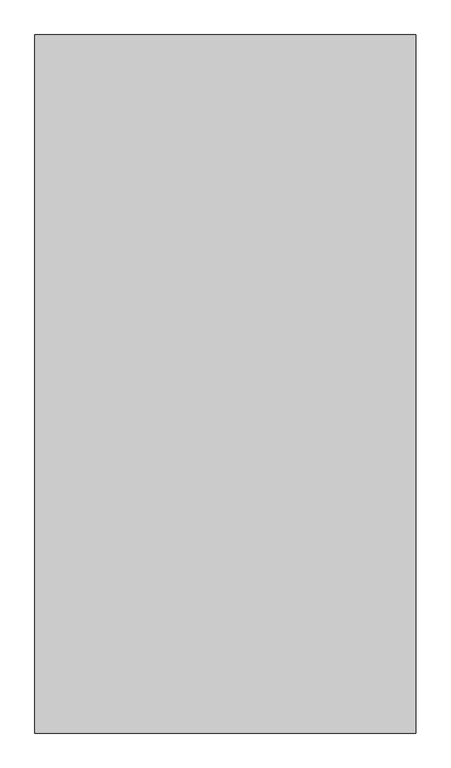
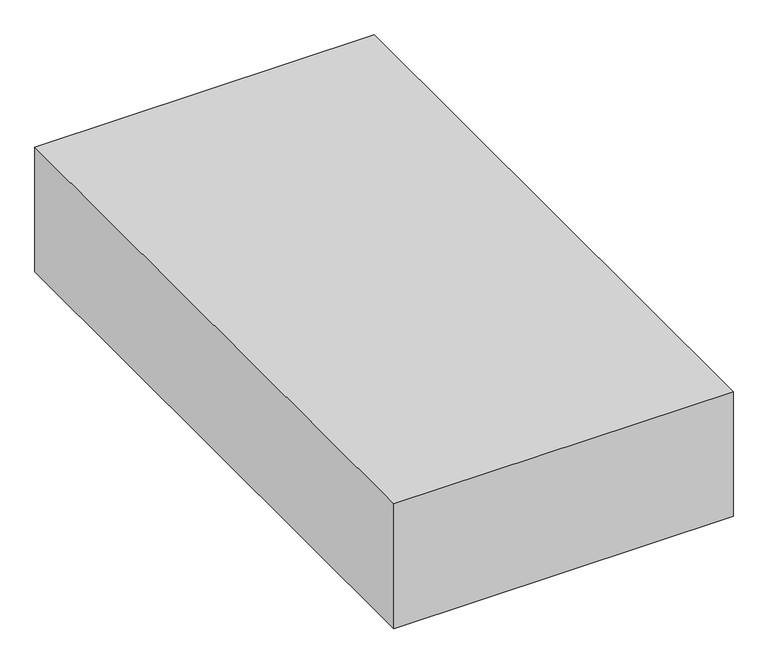
"""IFC4 building model written with IfcOpenShell, lengths in millimetres: proxy geometry, Space Planning Box_hec : Space Planning Box_hec."""

import ifcopenshell
import ifcopenshell.guid

model = None  # the IFC model being written
_history = None  # IfcOwnerHistory: only IFC2X3 demands one
_inside = {}  # id of a spatial element -> (the spatial element, [elements in it])
_under = {}  # id of a project, library or spatial element -> (it, [spatial elements below it])
_declared = {}  # id of a project -> (the project, [libraries it declares])
_typed = {}  # id of a type object -> (the type object, [elements of that type])
_made_of = {}  # id of a material, layer set ... -> (it, [elements and type objects made of it])


def new_model(schema):
    """Start an empty IFC model of exactly this schema.

    Asked for "IFC4X3", IfcOpenShell would pick the latest addendum, in which some entities
    have other attributes; the version numbers below select the first issue.
    IFC2X3 requires an IfcOwnerHistory on every rooted entity: one is made here for all.
    """
    global model, _history
    if schema == "IFC4X3":
        model = ifcopenshell.file(schema_version=(4, 3, 0, 0))
    else:
        model = ifcopenshell.file(schema=schema)
    _inside.clear()
    _under.clear()
    _declared.clear()
    _typed.clear()
    _made_of.clear()
    _history = None
    if model.schema == "IFC2X3":
        org = make("IfcOrganization", Name="unknown")
        user = make(
            "IfcPersonAndOrganization",
            ThePerson=make("IfcPerson", FamilyName="unknown"),
            TheOrganization=org,
        )
        app = make(
            "IfcApplication",
            ApplicationDeveloper=org,
            Version="unknown",
            ApplicationFullName="unknown",
            ApplicationIdentifier="unknown",
        )
        _history = make(
            "IfcOwnerHistory",
            OwningUser=user,
            OwningApplication=app,
            ChangeAction="ADDED",
            CreationDate=0,
        )
    return model


def make(cls, **values):
    """One entity of the class cls with the attributes given. An attribute that is None is left unset."""
    return model.create_entity(
        cls, **{name: value for name, value in values.items() if value is not None}
    )


def rooted(cls, **values):
    """An entity with a GlobalId (a new one), such as an element, a storey or a relation."""
    return make(cls, GlobalId=ifcopenshell.guid.new(), OwnerHistory=_history, **values)


def si_unit(unit_type, name, prefix=None):
    """IfcSIUnit, for example si_unit("LENGTHUNIT", "METRE", prefix="MILLI")."""
    return make("IfcSIUnit", UnitType=unit_type, Prefix=prefix, Name=name)


def assignment(units):
    """IfcUnitAssignment: the units of a project."""
    return None if units is None else make("IfcUnitAssignment", Units=units)


def point(xyz):
    """IfcCartesianPoint."""
    return None if xyz is None else make("IfcCartesianPoint", Coordinates=xyz)


def direction(xyz):
    """IfcDirection."""
    return None if xyz is None else make("IfcDirection", DirectionRatios=xyz)


def frame(location, z_axis=None, x_axis=None):
    """IfcAxis2Placement3D, a coordinate frame: its origin and axes. An axis left out is left unset."""
    return make(
        "IfcAxis2Placement3D",
        Location=point(location),
        Axis=direction(z_axis),
        RefDirection=direction(x_axis),
    )


def origin():
    """The frame at (0, 0, 0) with its axes left unset."""
    return frame((0.0, 0.0, 0.0))


def origin_with_axes():
    """The frame at (0, 0, 0) with the z axis (0, 0, 1) and the x axis (1, 0, 0) written out."""
    return frame((0.0, 0.0, 0.0), z_axis=(0.0, 0.0, 1.0), x_axis=(1.0, 0.0, 0.0))


def place(relative_to, where):
    """IfcLocalPlacement: puts the frame where relative to a parent placement (None: the world)."""
    return make(
        "IfcLocalPlacement", PlacementRelTo=relative_to, RelativePlacement=where
    )


def context(
    kind, dimensions, precision=None, world=None, true_north=None, identifier=None
):
    """IfcGeometricRepresentationContext, for example the 3D "Model" context."""
    return make(
        "IfcGeometricRepresentationContext",
        ContextIdentifier=identifier,
        ContextType=kind,
        CoordinateSpaceDimension=dimensions,
        Precision=precision,
        WorldCoordinateSystem=world,
        TrueNorth=true_north,
    )


def project(units=None, contexts=None):
    """IfcProject with its units and contexts."""
    return rooted(
        "IfcProject",
        Name="project",
        RepresentationContexts=contexts,
        UnitsInContext=assignment(units),
    )


def spatial(cls, under=None, at=None, **own):
    """A site, building, storey or space (cls), placed at a placement, below another one or the project."""
    s = rooted(cls, ObjectPlacement=at, **own)
    if under is not None:
        _under.setdefault(under.id(), (under, []))[1].append(s)
    return s


def polyline(points):
    """IfcPolyline through the points."""
    return make("IfcPolyline", Points=[point(p) for p in points])


def outline(outer, holes=None, kind="AREA"):
    """IfcArbitraryClosedProfileDef: a profile drawn as a closed curve; with holes, ...WithVoids."""
    if holes is None:
        return make("IfcArbitraryClosedProfileDef", ProfileType=kind, OuterCurve=outer)
    return make(
        "IfcArbitraryProfileDefWithVoids",
        ProfileType=kind,
        OuterCurve=outer,
        InnerCurves=holes,
    )


def extrude(swept, where, along, depth):
    """IfcExtrudedAreaSolid: the profile swept, set in the frame where, extruded along a direction by depth."""
    return make(
        "IfcExtrudedAreaSolid",
        SweptArea=swept,
        Position=where,
        ExtrudedDirection=direction(along),
        Depth=depth,
    )


def shape(context_of_items, identifier, shape_type, items):
    """IfcShapeRepresentation: the items that make up one representation, for example the "Body"."""
    return make(
        "IfcShapeRepresentation",
        ContextOfItems=context_of_items,
        RepresentationIdentifier=identifier,
        RepresentationType=shape_type,
        Items=items,
    )


def source(mapping_origin, context_of_items, identifier, shape_type, items):
    """IfcRepresentationMap: a shape defined once, which mapped items show again and again."""
    return make(
        "IfcRepresentationMap",
        MappingOrigin=mapping_origin,
        MappedRepresentation=shape(context_of_items, identifier, shape_type, items),
    )


def transform(
    local_origin,
    x_axis=None,
    y_axis=None,
    z_axis=None,
    scale=None,
    scale2=None,
    scale3=None,
    uniform=True,
):
    """IfcCartesianTransformationOperator3D, or its non-uniform kind. x_axis, y_axis, z_axis: its Axis1, 2, 3."""
    if uniform:
        return make(
            "IfcCartesianTransformationOperator3D",
            Axis1=direction(x_axis),
            Axis2=direction(y_axis),
            LocalOrigin=point(local_origin),
            Scale=scale,
            Axis3=direction(z_axis),
        )
    return make(
        "IfcCartesianTransformationOperator3DnonUniform",
        Axis1=direction(x_axis),
        Axis2=direction(y_axis),
        LocalOrigin=point(local_origin),
        Scale=scale,
        Axis3=direction(z_axis),
        Scale2=scale2,
        Scale3=scale3,
    )


def mapped(mapping_source, mapping_target):
    """IfcMappedItem: shows the shape of a source again, moved by a transform."""
    return make(
        "IfcMappedItem", MappingSource=mapping_source, MappingTarget=mapping_target
    )


def made_of(thing, what):
    """Note that an element or type object is made of a material, layer set ...; save() writes the relation."""
    if what is not None:
        _made_of.setdefault(what.id(), (what, []))[1].append(thing)
    return thing


def element(
    cls,
    number,
    at=None,
    inside=None,
    cuts=None,
    type_object=None,
    material=None,
    context=None,
    identifier="Body",
    shape_type=None,
    held_by="IfcProductDefinitionShape",
    body=None,
    shapes=None,
    **own,
):
    """One element of the class cls, such as IfcWall. Its Tag is "e" and its number.

    at: its placement. inside: the storey or other place that contains it. cuts: it is an
    opening in that element (IfcRelVoidsElement). A single representation is given by context,
    identifier, shape_type and body (its items); several are given by shapes. held_by: the class
    of the entity that holds the representations. save() writes the other relations.
    """
    e = rooted(cls, Tag="e%d" % number, ObjectPlacement=at, **own)
    if body is not None:
        shapes = [shape(context, identifier, shape_type, body)]
    if shapes is not None:
        e.Representation = make(held_by, Representations=shapes)
    if inside is not None:
        _inside.setdefault(inside.id(), (inside, []))[1].append(e)
    if cuts is not None:
        rooted(
            "IfcRelVoidsElement", RelatingBuildingElement=cuts, RelatedOpeningElement=e
        )
    if type_object is not None:
        _typed.setdefault(type_object.id(), (type_object, []))[1].append(e)
    return made_of(e, material)


def aggregate(whole, parts):
    """IfcRelAggregates: a whole, such as a stair, and the parts it consists of."""
    return rooted("IfcRelAggregates", RelatingObject=whole, RelatedObjects=parts)


def save(model, path):
    """Write the relations noted so far, then the file.

    IfcRelAggregates (storeys below a building ...), IfcRelContainedInSpatialStructure (elements
    in a storey), IfcRelDefinesByType, IfcRelAssociatesMaterial and IfcRelDeclares: one each for
    every whole, place, type object, material and project.
    """
    for whole, parts in _under.values():
        aggregate(whole, parts)
    for where, things in _inside.values():
        rooted(
            "IfcRelContainedInSpatialStructure",
            RelatedElements=things,
            RelatingStructure=where,
        )
    for kind, things in _typed.values():
        rooted("IfcRelDefinesByType", RelatedObjects=things, RelatingType=kind)
    for what, things in _made_of.values():
        rooted("IfcRelAssociatesMaterial", RelatedObjects=things, RelatingMaterial=what)
    for by, libraries in _declared.values():
        rooted("IfcRelDeclares", RelatingContext=by, RelatedDefinitions=libraries)
    model.write(path)


def generic_models_f0561c1d(model_context):
    return source(origin(), model_context, "Body", "SweptSolid", [
        extrude(outline(polyline([(4500.0, 8250.0), (4500.0, -8250.0), (-4500.0, -8250.0), (-4500.0, 8250.0), (4500.0, 8250.0)])), origin_with_axes(), (0.0, 0.0, 1.0), 3500.0),
    ])


if __name__ == "__main__":
    model = new_model("IFC4")
    model_context = context("Model", 3, world=origin())
    ifc_project = project(units=[si_unit("LENGTHUNIT", "METRE", prefix="MILLI")], contexts=[model_context])
    site = spatial("IfcSite", under=ifc_project)
    building = spatial("IfcBuilding", under=site)
    placement = place(None, origin())
    generic_models_shape = generic_models_f0561c1d(model_context)
    element("IfcBuildingElementProxy", 1, Name="Space Planning Box_hec : Space Planning Box_hec", ObjectType="Space Planning Box_hec : Space Planning Box_hec", at=placement, inside=building, context=model_context, shape_type="MappedRepresentation", body=[
        mapped(generic_models_shape, transform((0.0, 0.0, 0.0), x_axis=(1.0, 0.0, 0.0), y_axis=(0.0, 1.0, 0.0), z_axis=(0.0, 0.0, 1.0))),
    ])
    save(model, "model.ifc")

# Revit data of these elements
# Type "Space Planning Box_hec : Space Planning Box_hec"
#   Type Comments = "..."
#   Room Name [instance default] = "?"
#   Interior Finish [instance default] = ""
#   Exterior Finish [instance default] = ""
#   Department [instance default] = ""
#   Assembly Code = "..."
#   ceiling height [instance default] = 0
#   Width [instance default] = 1524 mm
#   Program Area [instance default] = 0.00 m²
#   Length [instance default] = 1524 mm
#   Height [instance default] = 1524 mm
#   Area [instance default] = 2.32258 m²
#   Fill Color [instance default] = Cyan
#   Default Elevation = 0
# Element 1 (IfcBuildingElementProxy, "Space Planning Box_hec : Space Planning Box_hec")
#   Room Name = "Open Office"
#   Exterior Finish = "RF1..N/A,,EW1..N/A..N/A"
#   Department = "HV"
#   Width = 9000 mm
#   Program Area = 148.50 m²
#   Length = 16500 mm
#   Height = 3500 mm
#   Area = 148.50 m²
#   Fill Color = Lime
#   Materials on its faces: "Lime"
# Materials
#   "Cyan": class "Generic", colour RGB 0 255 255, transparency 0.2, Cost = 0
#   "Lime": class "Generic", colour RGB 0 255 0, transparency 0.2, Cost = 0
